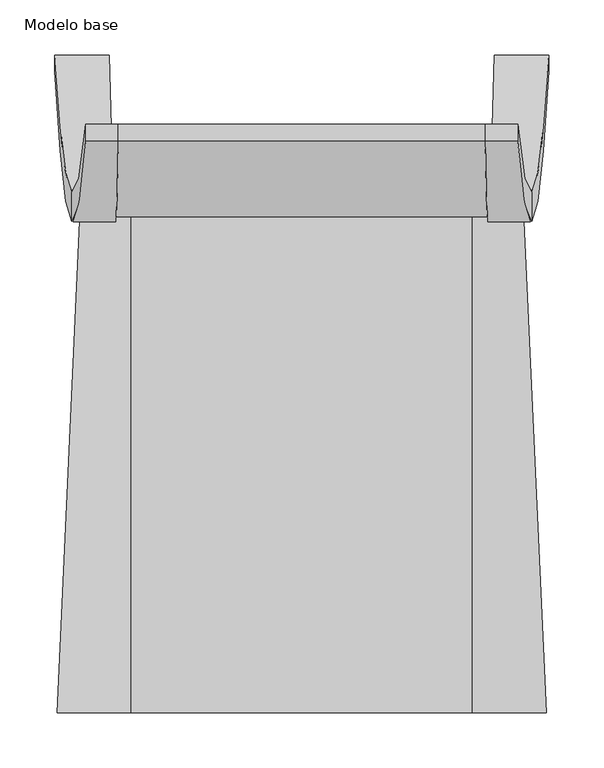
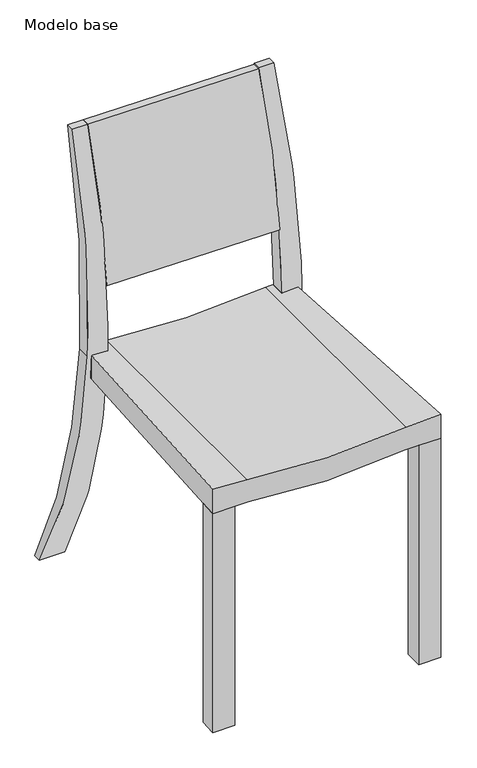
"""IFC4 building model written with IfcOpenShell, lengths in millimetres: furniture geometry, Silla - Madera (2) : Modelo base."""

from ifc_helpers import new_model, si_unit, frame, origin, origin_with_axes, place, context, project, spatial, polyline, circle_curve, ellipse_curve, outline, extrude, source, transform, mapped, element, save
from ifc_brep_helpers import plane_surface, cylinder_surface, revolved_surface, advanced_brep


def modelo_base_cd773059(model_context):
    return source(origin(), model_context, "Body", "SolidModel", [
        advanced_brep(
        [(-167.062, 520.2637315, 922.805277), (-167.062, 535.7344232, 922.805277), (-169.1260061, 476.85094, 631.1538985), (-169.1260061, 451.6822204, 631.1538985), (169.1428344, 451.6822204, 628.7599824), (167.0777417, 520.2637315, 920.4405823), (169.1428344, 476.85094, 628.7599824), (167.0777417, 535.7344232, 920.4405823)],
        [
            (0, 1),
            (1, 2, circle_curve(frame((-169.7736374, 1681.8941005, 539.6412969), z_axis=(0.9999749592362467, 0.0, -0.007076786026638103), x_axis=(-0.000231990271192452, -0.9994625301013882, -0.03278104793696645)), 1208.5131337)),
            (2, 3),
            (3, 0, circle_curve(frame((-169.8321061, 1530.470294, 531.3794559), z_axis=(-0.9999749592362468, 0.0, 0.007076786026638103), x_axis=(0.0025605874178329666, -0.9322444270823081, 0.36182008176171593)), 1083.3924247)),
            (3, 4),
            (4, 5, ellipse_curve(frame((169.8493062, 1530.470294, 528.975543), z_axis=(-0.9999749378861258, 0.0, -0.007079802231631731), x_axis=(0.007079802231623589, 0.0, -0.9999749378861258)), 1083.5009963, 1083.3924247)),
            (5, 0),
            (2, 6),
            (6, 4),
            (1, 7),
            (7, 6, ellipse_curve(frame((169.7908067, 1681.8941005, 537.2382119), z_axis=(0.9999749378861258, 0.0, 0.007079802231631731), x_axis=(-0.007079802231623589, 0.0, 0.9999749378861257)), 1208.6342443, 1208.5131337)),
            (5, 7),
        ],
        [
            plane_surface(frame((-167.0579851, 520.4837438, 923.3725916), z_axis=(-0.9999749592362468, 0.0, 0.007076786026638008), x_axis=(0.0065972943349872325, 0.3618291422397858, 0.9322210829698492))),
            cylinder_surface(frame((-169.8321061, 1530.470294, 531.3794559), z_axis=(0.9999749592362468, 0.0, -0.007076786026638103), x_axis=(0.0025605874178329666, -0.9322444270823081, 0.36182008176171593)), 1083.3924247),
            plane_surface(frame((184.488376, 451.6822204, 628.6513825), z_axis=(-0.007076786026638094, 0.0, -0.9999749592362467), x_axis=(-0.9999749592362467, 0.0, 0.007076786026638094))),
            revolved_surface(polyline([(-170.05400070707284, 474.03050623144077, 500.02496993185025), (186.61972368744534, 474.03050623144077, 497.50080309592073)]), (-169.7736374, 1681.8941005, 539.6412969), (-0.9999749592362467, 0.0, 0.007076786026638103)),
            plane_surface(frame((186.552382, 535.7344232, 920.302761), z_axis=(0.007076786026638094, 0.0, 0.9999749592362467), x_axis=(-0.9999749592362467, 0.0, 0.007076786026638094))),
            plane_surface(frame((167.061, -43.0, 922.8052375), z_axis=(0.9999749378861258, 0.0, 0.007079802231631731), x_axis=(0.0, 1.0, 0.0))),
        ],
        [
            (0, [[1, 2, 3, 4]]),
            (1, [[-4, 5, 6, 7]]),
            (2, [[-3, 8, 9, -5]]),
            (3, [[-2, 10, 11, -8]]),
            (4, [[-1, -7, 12, -10]]),
            (5, [[-6, -9, -11, -12]]),
        ],
    ),
        advanced_brep(
        [(224.9236272, 584.1809027, 3.307), (175.2970931, 584.1809027, 3.307), (175.2970931, 598.919, 3.307), (224.9236272, 598.919, 3.307), (170.0540007, 474.0305027, 500.0249699), (167.062, 535.7344266, 922.805275), (196.7208922, 535.7344266, 922.805275), (209.6209787, 473.9604495, 502.2216956), (209.6209787, 447.4551966, 502.2216956), (196.7208922, 520.483749, 922.805275), (167.062, 520.483749, 922.805275), (170.0540007, 447.5154198, 500.0249699)],
        [
            (0, 1),
            (1, 2),
            (2, 3),
            (3, 0),
            (2, 4, ellipse_curve(frame((169.6358332, 1681.8359776, 539.6411561), z_axis=(-0.9999442956654316, 0.0, -0.010554883522048576), x_axis=(-0.010554883522032881, 0.0, 0.9999442956654316)), 1208.5223284, 1208.4550084)),
            (4, 5, ellipse_curve(frame((169.7736384, 1681.8359776, 539.6411561), z_axis=(-0.9999749592362469, 0.0, -0.007076786026603054), x_axis=(-0.007076786026602528, 0.0, 0.9999749592362469)), 1208.4852698, 1208.4550084)),
            (5, 6),
            (6, 7, ellipse_curve(frame((208.4732537, 1681.8359776, 539.6411561), z_axis=(0.999529949707532, 0.0, 0.03065745647731723), x_axis=(-0.03065745647731804, 0.0, 0.9995299497075321)), 1209.0233102, 1208.4550084)),
            (7, 3, ellipse_curve(frame((208.4732537, 1681.8359776, 539.6411561), z_axis=(0.999529949707532, 0.0, 0.03065745647731721), x_axis=(-0.03065745647731806, 0.0, 0.999529949707532)), 1209.0233102, 1208.4550084)),
            (0, 8, ellipse_curve(frame((208.7440626, 1530.4189519, 530.8119297), z_axis=(-0.999529949707532, 0.0, -0.03065745647731721), x_axis=(0.03065745647731806, 0.0, -0.999529949707532)), 1083.8505448, 1083.3410805)),
            (8, 9, ellipse_curve(frame((208.7440626, 1530.4189519, 530.8119297), z_axis=(-0.999529949707532, 0.0, -0.03065745647731723), x_axis=(0.03065745647731804, 0.0, -0.9995299497075321)), 1083.8505448, 1083.3410805)),
            (9, 10),
            (10, 11, ellipse_curve(frame((169.8361225, 1530.4189519, 530.8119297), z_axis=(0.9999749592362469, 0.0, 0.007076786026603054), x_axis=(0.007076786026602528, 0.0, -0.9999749592362469)), 1083.3682089, 1083.3410805)),
            (11, 1, ellipse_curve(frame((169.7290298, 1530.4189519, 530.8119297), z_axis=(0.9999442956654316, 0.0, 0.010554883522048576), x_axis=(0.010554883522032881, 0.0, -0.9999442956654316)), 1083.4014307, 1083.3410805)),
            (11, 4),
            (10, 5),
            (9, 6),
            (8, 7),
        ],
        [
            plane_surface(frame((269.6998521, 584.1809027, 3.307), z_axis=(0.0, 0.0, -1.0), x_axis=(-1.0, 0.0, 0.0))),
            revolved_surface(polyline([(156.8800207899621, 2890.290986, 539.6411561), (245.53883321251948, 2890.290986, 539.6411561)]), (-284.9147268, 1681.8359776, 539.6411561), (-1.0, 0.0, 0.0)),
            cylinder_surface(frame((-284.9147268, 1530.4189519, 530.8119297), z_axis=(1.0, 0.0, 0.0), x_axis=(0.0, 1.0, 0.0)), 1083.3410805),
            plane_surface(frame((175.332, -43.0, 0.0), z_axis=(-0.9999442956654316, 0.0, -0.010554883522048576), x_axis=(0.0, 1.0, 0.0))),
            plane_surface(frame((170.0540007, -43.0, 500.0249699), z_axis=(-0.9999749592362469, 0.0, -0.007076786026603054), x_axis=(0.0, 1.0, 0.0))),
            plane_surface(frame((167.062, -43.0, 922.805275), z_axis=(0.0, 0.0, 1.0), x_axis=(0.0, 1.0, 0.0))),
            plane_surface(frame((196.7208922, -43.0, 922.805275), z_axis=(0.999529949707532, 0.0, 0.03065745647731723), x_axis=(0.0, 1.0, 0.0))),
            plane_surface(frame((209.6209787, -43.0, 502.2216956), z_axis=(0.999529949707532, 0.0, 0.03065745647731721), x_axis=(0.0, 1.0, 0.0))),
        ],
        [
            (0, [[1, 2, 3, 4]]),
            (1, [[-3, 5, 6, 7, 8, 9]]),
            (2, [[-1, 10, 11, 12, 13, 14]]),
            (3, [[15, -5, -2, -14]]),
            (4, [[-15, -13, 16, -6]]),
            (5, [[-16, -12, 17, -7]]),
            (6, [[-17, -11, 18, -8]]),
            (7, [[-18, -10, -4, -9]]),
        ],
    ),
        advanced_brep(
        [(-175.2970931, 584.1809027, 3.307), (-224.9236272, 584.1809027, 3.307), (-224.9236272, 598.919, 3.307), (-175.2970931, 598.919, 3.307), (-209.6209787, 473.9604495, 502.2216956), (-196.7208922, 535.7344266, 922.805275), (-167.062, 535.7344266, 922.805275), (-170.0540007, 474.0305027, 500.0249699), (-170.0540007, 447.5154198, 500.0249699), (-167.062, 520.483749, 922.805275), (-196.7208922, 520.483749, 922.805275), (-209.6209787, 447.4551966, 502.2216956)],
        [
            (0, 1),
            (1, 2),
            (2, 3),
            (3, 0),
            (2, 4, ellipse_curve(frame((-208.4732537, 1681.8359776, 539.6411561), z_axis=(-0.999529949707532, 0.0, 0.03065745647731722), x_axis=(-0.030657456477318046, 0.0, -0.999529949707532)), 1209.0233102, 1208.4550084)),
            (4, 5, ellipse_curve(frame((-208.4732537, 1681.8359776, 539.6411561), z_axis=(-0.999529949707532, 0.0, 0.030657456477317213), x_axis=(-0.030657456477318053, 0.0, -0.9995299497075318)), 1209.0233102, 1208.4550084)),
            (5, 6),
            (6, 7, ellipse_curve(frame((-169.7736384, 1681.8359776, 539.6411561), z_axis=(0.9999749592362467, 0.0, -0.007076786026638007), x_axis=(-0.007076786026630329, 0.0, -0.9999749592362467)), 1208.4852698, 1208.4550084)),
            (7, 3, ellipse_curve(frame((-169.6358332, 1681.8359776, 539.6411561), z_axis=(0.9999442956654323, 0.0, -0.010554883521987864), x_axis=(-0.010554883521967373, 0.0, -0.9999442956654325)), 1208.5223284, 1208.4550084)),
            (0, 8, ellipse_curve(frame((-169.7290298, 1530.4189519, 530.8119297), z_axis=(-0.9999442956654323, 0.0, 0.010554883521987864), x_axis=(0.010554883521967373, 0.0, 0.9999442956654325)), 1083.4014307, 1083.3410805)),
            (8, 9, ellipse_curve(frame((-169.8361225, 1530.4189519, 530.8119297), z_axis=(-0.9999749592362467, 0.0, 0.007076786026638007), x_axis=(0.007076786026630329, 0.0, 0.9999749592362467)), 1083.3682089, 1083.3410805)),
            (9, 10),
            (10, 11, ellipse_curve(frame((-208.7440626, 1530.4189519, 530.8119297), z_axis=(0.999529949707532, 0.0, -0.030657456477317213), x_axis=(0.030657456477318053, 0.0, 0.9995299497075318)), 1083.8505448, 1083.3410805)),
            (11, 1, ellipse_curve(frame((-208.7440626, 1530.4189519, 530.8119297), z_axis=(0.999529949707532, 0.0, -0.03065745647731722), x_axis=(0.030657456477318046, 0.0, 0.999529949707532)), 1083.8505448, 1083.3410805)),
            (4, 11),
            (10, 5),
            (9, 6),
            (8, 7),
        ],
        [
            plane_surface(frame((269.6998521, 584.1809027, 3.307), z_axis=(0.0, 0.0, -1.0), x_axis=(-1.0, 0.0, 0.0))),
            revolved_surface(polyline([(-245.53883321251948, 2890.290986, 539.6411561), (-156.88002079004121, 2890.290986, 539.6411561)]), (-284.9147268, 1681.8359776, 539.6411561), (-1.0, 0.0, 0.0)),
            cylinder_surface(frame((-284.9147268, 1530.4189519, 530.8119297), z_axis=(1.0, 0.0, 0.0), x_axis=(0.0, 1.0, 0.0)), 1083.3410805),
            plane_surface(frame((-209.6209787, -43.0, 502.2216956), z_axis=(-0.999529949707532, 0.0, 0.030657456477317213), x_axis=(0.0, 1.0, 0.0))),
            plane_surface(frame((-196.7208922, -43.0, 922.805275), z_axis=(0.0, 0.0, 1.0), x_axis=(0.0, 1.0, 0.0))),
            plane_surface(frame((-167.062, -43.0, 922.805275), z_axis=(0.9999749592362467, 0.0, -0.007076786026638007), x_axis=(0.0, 1.0, 0.0))),
            plane_surface(frame((-170.0540007, -43.0, 500.0249699), z_axis=(0.9999442956654323, 0.0, -0.010554883521987864), x_axis=(0.0, 1.0, 0.0))),
            plane_surface(frame((-230.4680491, -43.0, -177.4586702), z_axis=(-0.999529949707532, 0.0, 0.03065745647731722), x_axis=(0.0, 1.0, 0.0))),
        ],
        [
            (0, [[1, 2, 3, 4]]),
            (1, [[-3, 5, 6, 7, 8, 9]]),
            (2, [[-1, 10, 11, 12, 13, 14]]),
            (3, [[15, -13, 16, -6]]),
            (4, [[-16, -12, 17, -7]]),
            (5, [[-17, -11, 18, -8]]),
            (6, [[-18, -10, -4, -9]]),
            (7, [[-15, -5, -2, -14]]),
        ],
    ),
        advanced_brep(
        [(-222.6457845, 0.0, 453.04), (-179.6457845, 0.0, 453.04), (-153.3625843, 0.0, 453.04), (153.3625843, 0.0, 453.04), (179.6457845, 0.0, 453.04), (222.6457845, 0.0, 453.04), (222.6457845, 0.0, 502.944822), (155.483, 0.0, 499.216), (-155.483, 0.0, 499.216), (-222.6457845, 0.0, 502.944822), (-155.483, 476.488, 499.216), (155.483, 476.488, 499.216), (200.7926448, 476.488, 501.7315539), (200.7926448, 476.488, 453.04), (179.6457845, 476.488, 453.04), (153.3625843, 476.488, 453.04), (-153.3625843, 476.488, 453.04), (-179.6457845, 476.488, 453.04), (-200.7915799, 476.488, 453.04), (-200.7915799, 476.488, 501.7314947), (-202.123, 447.459, 453.04), (202.124, 447.459, 453.04), (202.124, 447.459, 501.8054696), (-202.123, 447.459, 501.8054141)],
        [
            (0, 1),
            (1, 2),
            (2, 3, circle_curve(frame((0.0, 0.0, 1620.8639519), z_axis=(0.0, -1.0, 0.0), x_axis=(1.0, 0.0, 0.0)), 1177.8509519)),
            (3, 4),
            (4, 5),
            (5, 6),
            (6, 7),
            (7, 8, circle_curve(frame((0.0, 0.0, 1957.3962887), z_axis=(0.0, 1.0, 0.0), x_axis=(1.0, 0.0, 0.0)), 1466.4462887)),
            (8, 9),
            (9, 0),
            (10, 11, circle_curve(frame((0.0, 476.488, 1957.3962887), z_axis=(0.0, -1.0, 0.0), x_axis=(1.0, 0.0, 0.0)), 1466.4462887)),
            (11, 12),
            (12, 13),
            (13, 14),
            (14, 15),
            (15, 16, circle_curve(frame((0.0, 476.488, 1620.8639519), z_axis=(0.0, 1.0, 0.0), x_axis=(1.0, 0.0, 0.0)), 1177.8509519)),
            (16, 17),
            (17, 18),
            (18, 19),
            (19, 10),
            (0, 20),
            (20, 18),
            (17, 1),
            (16, 2),
            (15, 3),
            (14, 4),
            (13, 21),
            (21, 5),
            (6, 22),
            (22, 12),
            (11, 7),
            (10, 8),
            (19, 23),
            (23, 9),
            (20, 23),
            (22, 21),
        ],
        [
            plane_surface(frame((-222.6457845, 0.0, 453.04), z_axis=(0.0, -1.0, 0.0), x_axis=(0.0, 0.0, -1.0))),
            plane_surface(frame((-222.6457845, 476.488, 453.04), z_axis=(0.0, 1.0, 0.0), x_axis=(0.0, 0.0, 1.0))),
            plane_surface(frame((-222.6457845, 0.0, 453.04), z_axis=(0.0, 0.0, -1.0), x_axis=(0.0, 1.0, 0.0))),
            plane_surface(frame((-179.6457845, 0.0, 453.04), z_axis=(0.0, 0.0, -1.0), x_axis=(0.0, 1.0, 0.0))),
            cylinder_surface(frame((0.0, 476.488, 1620.8639519), z_axis=(0.0, -1.0, 0.0), x_axis=(1.0, 0.0, 0.0)), 1177.8509519),
            plane_surface(frame((153.3625843, 0.0, 453.04), z_axis=(0.0, 0.0, -1.0), x_axis=(0.0, 1.0, 0.0))),
            plane_surface(frame((179.6457845, 0.0, 453.04), z_axis=(0.0, 0.0, -1.0), x_axis=(0.0, 1.0, 0.0))),
            plane_surface(frame((222.6457845, 0.0, 502.944822), z_axis=(-0.055433801494316516, 0.0, 0.9984623646647323), x_axis=(0.0, 1.0, 0.0))),
            revolved_surface(polyline([(1466.4462887, 476.488, 1957.3962887), (1466.4462887, 0.0, 1957.3962887)]), (0.0, 476.488, 1957.3962887), (0.0, 1.0, 0.0)),
            plane_surface(frame((-155.483, 0.0, 499.216), z_axis=(0.055433801494308495, 0.0, 0.9984623646647327), x_axis=(0.0, 1.0, 0.0))),
            plane_surface(frame((-202.123, 447.459, 708.9557379), z_axis=(-0.9989498494941665, 0.04581700771091594, 0.0), x_axis=(0.0, 0.0, -1.0))),
            plane_surface(frame((193.8773396, 627.2699913, 708.9557379), z_axis=(0.998949951670504, 0.04581477990231496, 0.0), x_axis=(0.0, 0.0, -1.0))),
            plane_surface(frame((202.124, 447.459, 708.9557379), z_axis=(0.998949951670504, 0.045814779902315125, 0.0), x_axis=(0.0, 0.0, -1.0))),
            plane_surface(frame((-222.6457845, 0.0, 708.9557379), z_axis=(-0.9989498494941665, 0.04581700771091578, 0.0), x_axis=(0.0, 0.0, -1.0))),
        ],
        [
            (0, [[1, 2, 3, 4, 5, 6, 7, 8, 9, 10]]),
            (1, [[11, 12, 13, 14, 15, 16, 17, 18, 19, 20]]),
            (2, [[-1, 21, 22, -18, 23]]),
            (3, [[-2, -23, -17, 24]]),
            (4, [[-3, -24, -16, 25]]),
            (5, [[-4, -25, -15, 26]]),
            (6, [[-5, -26, -14, 27, 28]]),
            (7, [[-7, 29, 30, -12, 31]]),
            (8, [[-8, -31, -11, 32]]),
            (9, [[-9, -32, -20, 33, 34]]),
            (10, [[35, -33, -19, -22]]),
            (11, [[36, -27, -13, -30]]),
            (12, [[-36, -29, -6, -28]]),
            (13, [[-35, -21, -10, -34]]),
        ],
    ),
        extrude(outline(polyline([(-179.6457845, 34.744), (-179.6457845, 0.0), (-222.6457845, 0.0), (-221.0522449, 34.744), (-179.6457845, 34.744)])), origin_with_axes(), (0.0, 0.0, 1.0), 453.04),
        extrude(outline(polyline([(179.6457845, 0.0), (179.6457845, 34.744), (221.0523225, 34.744), (222.6457845, 0.0), (179.6457845, 0.0)])), origin_with_axes(), (0.0, 0.0, 1.0), 453.04),
    ])


if __name__ == "__main__":
    model = new_model("IFC4")
    model_context = context("Model", 3, world=origin())
    ifc_project = project(units=[si_unit("LENGTHUNIT", "METRE", prefix="MILLI")], contexts=[model_context])
    site = spatial("IfcSite", under=ifc_project)
    building = spatial("IfcBuilding", under=site)
    placement = place(None, origin())
    modelo_base_shape = modelo_base_cd773059(model_context)
    element("IfcFurniture", 1, ObjectType="Silla - Madera (2) : Modelo base", at=placement, inside=building, context=model_context, shape_type="MappedRepresentation", body=[
        mapped(modelo_base_shape, transform((0.0, 0.0, 0.0), x_axis=(1.0, 0.0, 0.0), y_axis=(0.0, 1.0, 0.0), z_axis=(0.0, 0.0, 1.0))),
    ])
    save(model, "model.ifc")

# Revit data of these elements
# Type "Silla - Madera (2) : Modelo base"
#   Máscara planta = yes
#   Máscara lateral = yes
#   Material = none
#   Manufacturer = ""
#   Default Elevation = 0
#   Assembly Code = ""
# Element 1 (IfcFurniture, "Silla - Madera (2) : Modelo base")
#   Materials on its faces: "Madera - Listel"
# Materials
#   "Madera - Listel": class "Madera", colour RGB 210 180 110, transparency 0, Cost = 0
